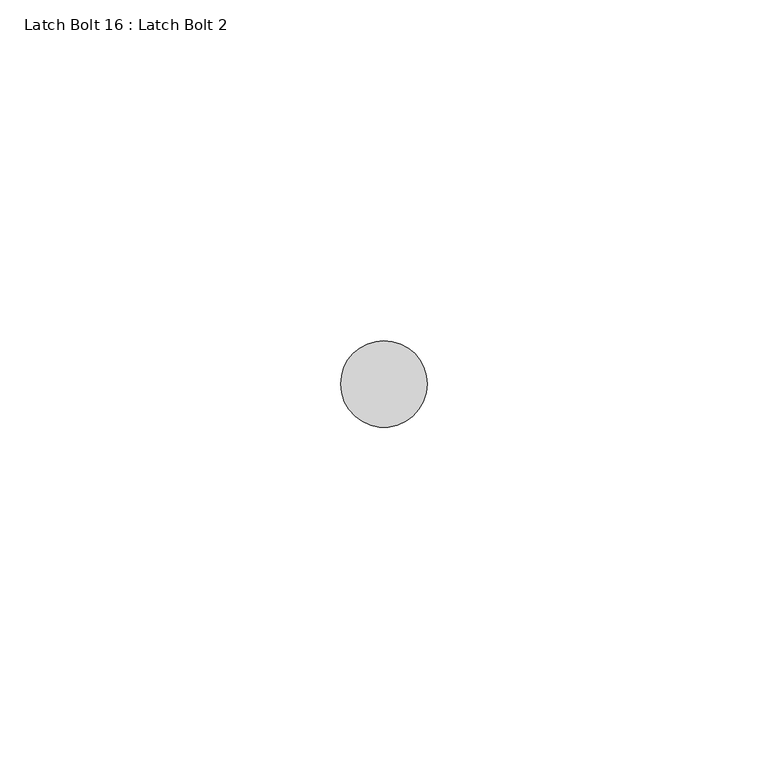
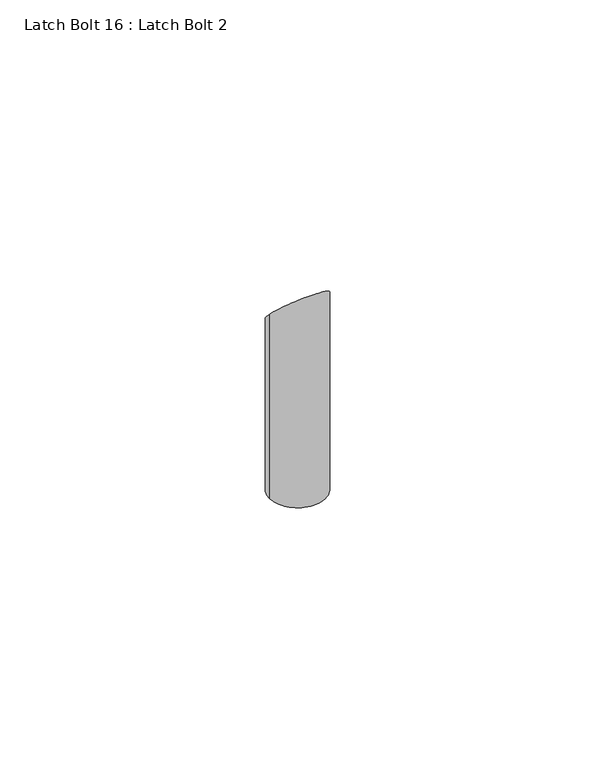
"""IFC4 building model written with IfcOpenShell, lengths in millimetres: proxy geometry, Latch Bolt 16 : Latch Bolt 2."""

from ifc_helpers import new_model, si_unit, frame, origin, place, context, project, spatial, circle_curve, ellipse_curve, source, transform, mapped, element, save
from ifc_brep_helpers import plane_surface, cylinder_surface, advanced_brep


def latch_bolt_16_latch_bolt_2_5f3dc6ce(model_context):
    return source(origin(), model_context, "Body", "AdvancedBrep", [
        advanced_brep(
        [(587306.3384816, -535293.641467, 1022.35), (587319.0384816, -535293.641467, 1022.35), (587319.0384816, -535293.641467, 1066.7505507), (587306.3384816, -535293.641467, 1066.7505507), (587312.6884816, -535287.291467, 1060.4005507)],
        [
            (0, 1, circle_curve(frame((587312.6884816, -535293.641467, 1022.35), z_axis=(0.0, 0.0, -1.0), x_axis=(1.0, 0.0, 0.0)), 6.35)),
            (1, 0, circle_curve(frame((587312.6884816, -535293.641467, 1022.35), z_axis=(0.0, 0.0, -1.0), x_axis=(1.0, 0.0, 0.0)), 6.35)),
            (1, 2),
            (2, 3, ellipse_curve(frame((587312.6884816, -535293.641467, 1066.7505507), z_axis=(0.0, -0.7071067811861375, -0.7071067811869577), x_axis=(0.0, -0.7071067811869577, 0.7071067811861372)), 8.9802561, 6.35)),
            (3, 0),
            (3, 4, ellipse_curve(frame((587312.6884816, -535293.641467, 1066.7505507), z_axis=(0.0, -0.7071067811861375, -0.7071067811869577), x_axis=(0.0, -0.7071067811869577, 0.7071067811861372)), 8.9802561, 6.35)),
            (4, 2, ellipse_curve(frame((587312.6884816, -535293.641467, 1066.7505507), z_axis=(0.0, -0.7071067811861375, -0.7071067811869577), x_axis=(0.0, -0.7071067811869577, 0.7071067811861372)), 8.9802561, 6.35)),
        ],
        [
            plane_surface(frame((587319.0384816, -535293.641467, 1022.35), z_axis=(0.0, 0.0, -1.0), x_axis=(0.0, -1.0, 0.0))),
            cylinder_surface(frame((587312.6884816, -535293.641467, 1022.35), z_axis=(0.0, 0.0, 1.0), x_axis=(1.0, 0.0, 0.0)), 6.35),
            plane_surface(frame((587338.1185739, -535303.166467, 1076.2755507), z_axis=(0.0, 0.7071067811861375, 0.7071067811869577), x_axis=(-1.0, 0.0, 0.0))),
        ],
        [
            (0, [[1, 2]]),
            (1, [[-2, 3, 4, 5]]),
            (1, [[-1, -5, 6, 7, -3]]),
            (2, [[-4, -7, -6]]),
        ],
    ),
    ])


if __name__ == "__main__":
    model = new_model("IFC4")
    model_context = context("Model", 3, world=origin())
    ifc_project = project(units=[si_unit("LENGTHUNIT", "METRE", prefix="MILLI")], contexts=[model_context])
    site = spatial("IfcSite", under=ifc_project)
    building = spatial("IfcBuilding", under=site)
    placement = place(None, origin())
    latch_bolt_16_latch_bolt_2_shape = latch_bolt_16_latch_bolt_2_5f3dc6ce(model_context)
    element("IfcBuildingElementProxy", 1, Name="Latch Bolt 16 : Latch Bolt 2", ObjectType="Latch Bolt 16 : Latch Bolt 2", at=placement, inside=building, context=model_context, shape_type="MappedRepresentation", body=[
        mapped(latch_bolt_16_latch_bolt_2_shape, transform((0.0, 0.0, 0.0), x_axis=(1.0, 0.0, 0.0), y_axis=(0.0, 1.0, 0.0), z_axis=(0.0, 0.0, 1.0))),
    ])
    save(model, "model.ifc")

# Revit data of these elements
# Element 1 (IfcBuildingElementProxy, "Latch Bolt 16 : Latch Bolt 2")
#   Materials on its faces: "GALV. GATE LATCH"
# Materials
#   "GALV. GATE LATCH": class "Metal", colour RGB 189 187 185, transparency 0, Description = "Carbon steel", Cost = 0
